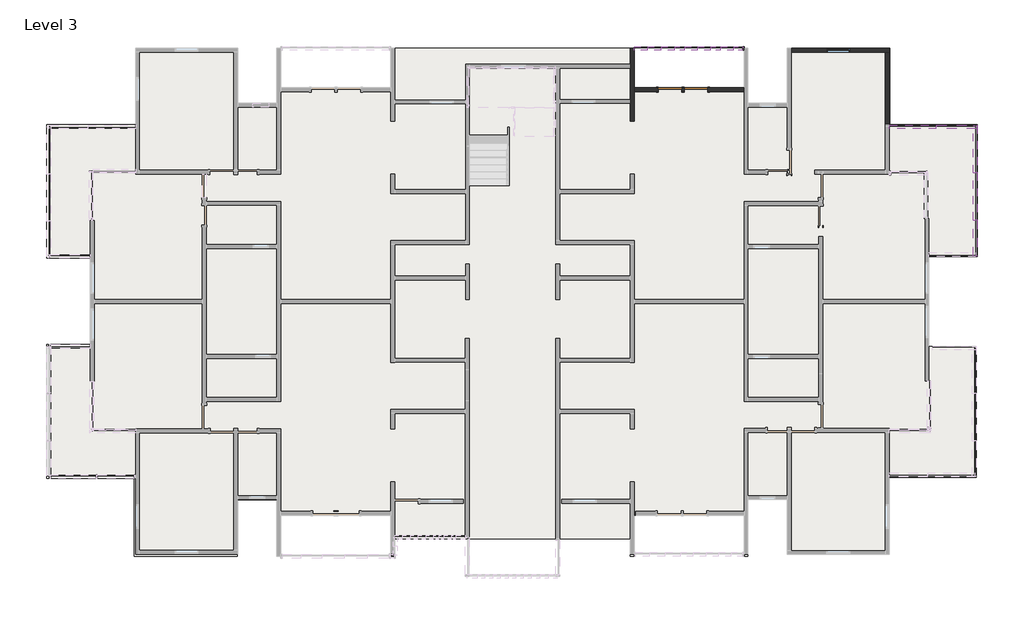
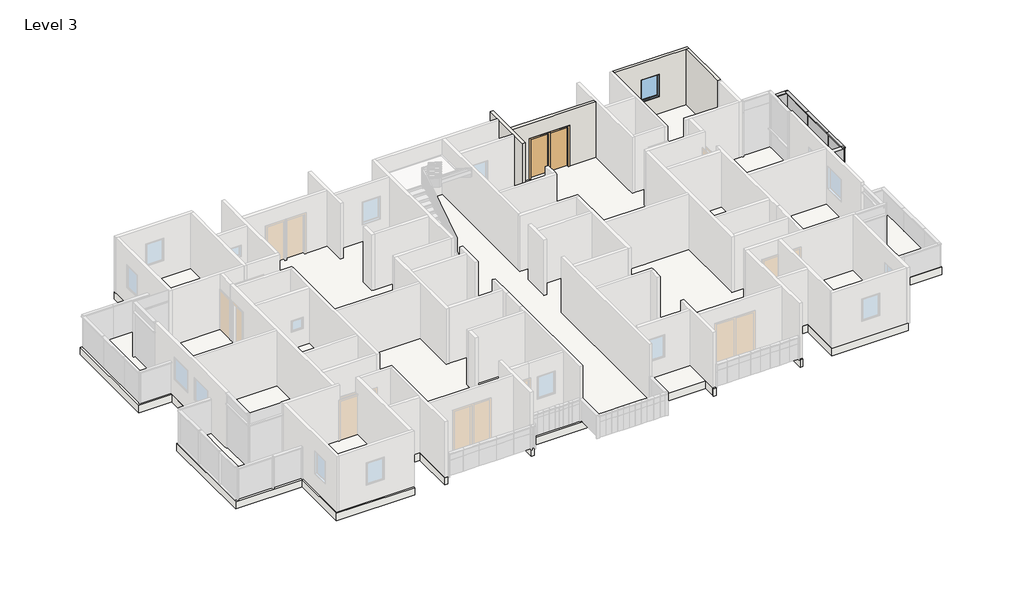
# One storey, part 5 of 7: 15 members, 14 plates, 4 walls, 2 doors, 1 slab, 1 window.
"""IFC4 building model written with IfcOpenShell, lengths in millimetres."""

import ifcopenshell
import ifcopenshell.guid

model = None  # the IFC model being written
_history = None  # IfcOwnerHistory: only IFC2X3 demands one
_inside = {}  # id of a spatial element -> (the spatial element, [elements in it])
_under = {}  # id of a project, library or spatial element -> (it, [spatial elements below it])
_declared = {}  # id of a project -> (the project, [libraries it declares])
_typed = {}  # id of a type object -> (the type object, [elements of that type])
_made_of = {}  # id of a material, layer set ... -> (it, [elements and type objects made of it])


def new_model(schema):
    """Start an empty IFC model of exactly this schema.

    Asked for "IFC4X3", IfcOpenShell would pick the latest addendum, in which some entities
    have other attributes; the version numbers below select the first issue.
    IFC2X3 requires an IfcOwnerHistory on every rooted entity: one is made here for all.
    """
    global model, _history
    if schema == "IFC4X3":
        model = ifcopenshell.file(schema_version=(4, 3, 0, 0))
    else:
        model = ifcopenshell.file(schema=schema)
    _inside.clear()
    _under.clear()
    _declared.clear()
    _typed.clear()
    _made_of.clear()
    _history = None
    if model.schema == "IFC2X3":
        org = make("IfcOrganization", Name="unknown")
        user = make(
            "IfcPersonAndOrganization",
            ThePerson=make("IfcPerson", FamilyName="unknown"),
            TheOrganization=org,
        )
        app = make(
            "IfcApplication",
            ApplicationDeveloper=org,
            Version="unknown",
            ApplicationFullName="unknown",
            ApplicationIdentifier="unknown",
        )
        _history = make(
            "IfcOwnerHistory",
            OwningUser=user,
            OwningApplication=app,
            ChangeAction="ADDED",
            CreationDate=0,
        )
    return model


def make(cls, **values):
    """One entity of the class cls with the attributes given. An attribute that is None is left unset."""
    return model.create_entity(
        cls, **{name: value for name, value in values.items() if value is not None}
    )


def rooted(cls, **values):
    """An entity with a GlobalId (a new one), such as an element, a storey or a relation."""
    return make(cls, GlobalId=ifcopenshell.guid.new(), OwnerHistory=_history, **values)


def si_unit(unit_type, name, prefix=None):
    """IfcSIUnit, for example si_unit("LENGTHUNIT", "METRE", prefix="MILLI")."""
    return make("IfcSIUnit", UnitType=unit_type, Prefix=prefix, Name=name)


def assignment(units):
    """IfcUnitAssignment: the units of a project."""
    return None if units is None else make("IfcUnitAssignment", Units=units)


def point(xyz):
    """IfcCartesianPoint."""
    return None if xyz is None else make("IfcCartesianPoint", Coordinates=xyz)


def direction(xyz):
    """IfcDirection."""
    return None if xyz is None else make("IfcDirection", DirectionRatios=xyz)


def frame(location, z_axis=None, x_axis=None):
    """IfcAxis2Placement3D, a coordinate frame: its origin and axes. An axis left out is left unset."""
    return make(
        "IfcAxis2Placement3D",
        Location=point(location),
        Axis=direction(z_axis),
        RefDirection=direction(x_axis),
    )


def origin():
    """The frame at (0, 0, 0) with its axes left unset."""
    return frame((0.0, 0.0, 0.0))


def origin_with_axes():
    """The frame at (0, 0, 0) with the z axis (0, 0, 1) and the x axis (1, 0, 0) written out."""
    return frame((0.0, 0.0, 0.0), z_axis=(0.0, 0.0, 1.0), x_axis=(1.0, 0.0, 0.0))


def place(relative_to, where):
    """IfcLocalPlacement: puts the frame where relative to a parent placement (None: the world)."""
    return make(
        "IfcLocalPlacement", PlacementRelTo=relative_to, RelativePlacement=where
    )


def context(
    kind, dimensions, precision=None, world=None, true_north=None, identifier=None
):
    """IfcGeometricRepresentationContext, for example the 3D "Model" context."""
    return make(
        "IfcGeometricRepresentationContext",
        ContextIdentifier=identifier,
        ContextType=kind,
        CoordinateSpaceDimension=dimensions,
        Precision=precision,
        WorldCoordinateSystem=world,
        TrueNorth=true_north,
    )


def project(units=None, contexts=None):
    """IfcProject with its units and contexts."""
    return rooted(
        "IfcProject",
        Name="project",
        RepresentationContexts=contexts,
        UnitsInContext=assignment(units),
    )


def spatial(cls, under=None, at=None, **own):
    """A site, building, storey or space (cls), placed at a placement, below another one or the project."""
    s = rooted(cls, ObjectPlacement=at, **own)
    if under is not None:
        _under.setdefault(under.id(), (under, []))[1].append(s)
    return s


def polyline(points):
    """IfcPolyline through the points."""
    return make("IfcPolyline", Points=[point(p) for p in points])


def outline(outer, holes=None, kind="AREA"):
    """IfcArbitraryClosedProfileDef: a profile drawn as a closed curve; with holes, ...WithVoids."""
    if holes is None:
        return make("IfcArbitraryClosedProfileDef", ProfileType=kind, OuterCurve=outer)
    return make(
        "IfcArbitraryProfileDefWithVoids",
        ProfileType=kind,
        OuterCurve=outer,
        InnerCurves=holes,
    )


def extrude(swept, where, along, depth):
    """IfcExtrudedAreaSolid: the profile swept, set in the frame where, extruded along a direction by depth."""
    return make(
        "IfcExtrudedAreaSolid",
        SweptArea=swept,
        Position=where,
        ExtrudedDirection=direction(along),
        Depth=depth,
    )


def faces_of(points, faces, orient=None, outer=None):
    """IfcFace entities. A face is a list of loops; a loop is a list of indices into points, from 0.

    orient and outer hold one flag for each loop. By default every Orientation is true, the
    first loop of a face is its IfcFaceOuterBound and the others are IfcFaceBound.
    """
    made = []
    for i, loops in enumerate(faces):
        bounds = []
        for j, loop in enumerate(loops):
            is_outer = j == 0 if outer is None else outer[i][j]
            bounds.append(
                make(
                    "IfcFaceOuterBound" if is_outer else "IfcFaceBound",
                    Bound=make("IfcPolyLoop", Polygon=[points[k] for k in loop]),
                    Orientation=True if orient is None else orient[i][j],
                )
            )
        made.append(make("IfcFace", Bounds=bounds))
    return made


def faceted_brep(points, faces, orient=None, outer=None, voids=None):
    """IfcFacetedBrep: a solid bounded by flat faces; with voids (closed shells), ...WithVoids."""
    shared = [point(p) for p in points]
    hull = make("IfcClosedShell", CfsFaces=faces_of(shared, faces, orient, outer))
    if voids is None:
        return make("IfcFacetedBrep", Outer=hull)
    return make(
        "IfcFacetedBrepWithVoids",
        Outer=hull,
        Voids=[
            make(cls, CfsFaces=faces_of(shared, fs, o, b)) for cls, fs, o, b in voids
        ],
    )


def shape(context_of_items, identifier, shape_type, items):
    """IfcShapeRepresentation: the items that make up one representation, for example the "Body"."""
    return make(
        "IfcShapeRepresentation",
        ContextOfItems=context_of_items,
        RepresentationIdentifier=identifier,
        RepresentationType=shape_type,
        Items=items,
    )


def source(mapping_origin, context_of_items, identifier, shape_type, items):
    """IfcRepresentationMap: a shape defined once, which mapped items show again and again."""
    return make(
        "IfcRepresentationMap",
        MappingOrigin=mapping_origin,
        MappedRepresentation=shape(context_of_items, identifier, shape_type, items),
    )


def transform(
    local_origin,
    x_axis=None,
    y_axis=None,
    z_axis=None,
    scale=None,
    scale2=None,
    scale3=None,
    uniform=True,
):
    """IfcCartesianTransformationOperator3D, or its non-uniform kind. x_axis, y_axis, z_axis: its Axis1, 2, 3."""
    if uniform:
        return make(
            "IfcCartesianTransformationOperator3D",
            Axis1=direction(x_axis),
            Axis2=direction(y_axis),
            LocalOrigin=point(local_origin),
            Scale=scale,
            Axis3=direction(z_axis),
        )
    return make(
        "IfcCartesianTransformationOperator3DnonUniform",
        Axis1=direction(x_axis),
        Axis2=direction(y_axis),
        LocalOrigin=point(local_origin),
        Scale=scale,
        Axis3=direction(z_axis),
        Scale2=scale2,
        Scale3=scale3,
    )


def mapped(mapping_source, mapping_target):
    """IfcMappedItem: shows the shape of a source again, moved by a transform."""
    return make(
        "IfcMappedItem", MappingSource=mapping_source, MappingTarget=mapping_target
    )


def made_of(thing, what):
    """Note that an element or type object is made of a material, layer set ...; save() writes the relation."""
    if what is not None:
        _made_of.setdefault(what.id(), (what, []))[1].append(thing)
    return thing


def element(
    cls,
    number,
    at=None,
    inside=None,
    cuts=None,
    type_object=None,
    material=None,
    context=None,
    identifier="Body",
    shape_type=None,
    held_by="IfcProductDefinitionShape",
    body=None,
    shapes=None,
    **own,
):
    """One element of the class cls, such as IfcWall. Its Tag is "e" and its number.

    at: its placement. inside: the storey or other place that contains it. cuts: it is an
    opening in that element (IfcRelVoidsElement). A single representation is given by context,
    identifier, shape_type and body (its items); several are given by shapes. held_by: the class
    of the entity that holds the representations. save() writes the other relations.
    """
    e = rooted(cls, Tag="e%d" % number, ObjectPlacement=at, **own)
    if body is not None:
        shapes = [shape(context, identifier, shape_type, body)]
    if shapes is not None:
        e.Representation = make(held_by, Representations=shapes)
    if inside is not None:
        _inside.setdefault(inside.id(), (inside, []))[1].append(e)
    if cuts is not None:
        rooted(
            "IfcRelVoidsElement", RelatingBuildingElement=cuts, RelatedOpeningElement=e
        )
    if type_object is not None:
        _typed.setdefault(type_object.id(), (type_object, []))[1].append(e)
    return made_of(e, material)


def aggregate(whole, parts):
    """IfcRelAggregates: a whole, such as a stair, and the parts it consists of."""
    return rooted("IfcRelAggregates", RelatingObject=whole, RelatedObjects=parts)


def save(model, path):
    """Write the relations noted so far, then the file.

    IfcRelAggregates (storeys below a building ...), IfcRelContainedInSpatialStructure (elements
    in a storey), IfcRelDefinesByType, IfcRelAssociatesMaterial and IfcRelDeclares: one each for
    every whole, place, type object, material and project.
    """
    for whole, parts in _under.values():
        aggregate(whole, parts)
    for where, things in _inside.values():
        rooted(
            "IfcRelContainedInSpatialStructure",
            RelatedElements=things,
            RelatingStructure=where,
        )
    for kind, things in _typed.values():
        rooted("IfcRelDefinesByType", RelatedObjects=things, RelatingType=kind)
    for what, things in _made_of.values():
        rooted("IfcRelAssociatesMaterial", RelatedObjects=things, RelatingMaterial=what)
    for by, libraries in _declared.values():
        rooted("IfcRelDeclares", RelatingContext=by, RelatedDefinitions=libraries)
    model.write(path)


def m_single_flush_0915_x_2134mm_138fd904(model_context):
    return source(origin(), model_context, "Body", "SweptSolid", [
        extrude(outline(polyline([(2210.0, -533.5), (0.0, -533.5), (0.0, -457.5), (2134.0, -457.5), (2134.0, 457.5), (0.0, 457.5), (0.0, 533.5), (2210.0, 533.5), (2210.0, -533.5)])), frame((0.0, 75.0, 0.0), z_axis=(0.0, 1.0, 0.0), x_axis=(0.0, 0.0, 1.0)), (0.0, 0.0, 1.0), 25.0),
        extrude(outline(polyline([(2210.0, 533.5), (2210.0, -533.5), (0.0, -533.5), (0.0, -457.5), (2134.0, -457.5), (2134.0, 457.5), (0.0, 457.5), (0.0, 533.5), (2210.0, 533.5)])), frame((0.0, -100.0, 0.0), z_axis=(0.0, 1.0, 0.0), x_axis=(0.0, 0.0, 1.0)), (0.0, 0.0, 1.0), 25.0),
        extrude(outline(polyline([(457.5, 24.0), (-457.5, 24.0), (-457.5, 75.0), (457.5, 75.0), (457.5, 24.0)])), origin_with_axes(), (0.0, 0.0, 1.0), 2134.0),
    ])


def rectangular_mullion_50mm_x_150mm_42770ee2(model_context):
    return source(origin(), model_context, "Body", "SweptSolid", [
        extrude(outline(polyline([(0.0, 75.0), (0.0, -75.0), (-50.0, -75.0), (-50.0, 75.0), (0.0, 75.0)])), frame((0.0, 0.0, -1830.0000003), z_axis=(0.0, 0.0, 1.0), x_axis=(1.0, 0.0, 0.0)), (0.0, 0.0, 1.0), 1830.0000003),
    ])


def rectangular_mullion_50mm_x_150mm_aaee7d48(model_context):
    return source(origin(), model_context, "Body", "SweptSolid", [
        extrude(outline(polyline([(0.0, 75.0), (0.0, -75.0), (-50.0, -75.0), (-50.0, 75.0), (0.0, 75.0)])), frame((0.0, 0.0, -1830.0), z_axis=(0.0, 0.0, 1.0), x_axis=(1.0, 0.0, 0.0)), (0.0, 0.0, 1.0), 1830.0),
    ])


def rectangular_mullion_50mm_x_150mm_efa02866(model_context):
    return source(origin(), model_context, "Body", "SweptSolid", [
        extrude(outline(polyline([(0.0, 75.0), (0.0, -75.0), (-50.0, -75.0), (-50.0, 75.0), (0.0, 75.0)])), frame((0.0, 0.0, -1399.9999997), z_axis=(0.0, 0.0, 1.0), x_axis=(1.0, 0.0, 0.0)), (0.0, 0.0, 1.0), 1399.9999997),
    ])


def rectangular_mullion_50mm_x_150mm_d9f1e9e9(model_context):
    return source(origin(), model_context, "Body", "SweptSolid", [
        extrude(outline(polyline([(0.0, 75.0), (0.0, -75.0), (-50.0, -75.0), (-50.0, 75.0), (0.0, 75.0)])), frame((0.0, 0.0, -1565.8160321), z_axis=(0.0, 0.0, 1.0), x_axis=(1.0, 0.0, 0.0)), (0.0, 0.0, 1.0), 1565.8160321),
    ])


def rectangular_mullion_50mm_x_150mm_729c0cfc(model_context):
    return source(origin(), model_context, "Body", "SweptSolid", [
        extrude(outline(polyline([(0.0, 75.0), (0.0, -75.0), (-50.0, -75.0), (-50.0, 75.0), (0.0, 75.0)])), frame((0.0, 0.0, -1250.0), z_axis=(0.0, 0.0, 1.0), x_axis=(1.0, 0.0, 0.0)), (0.0, 0.0, 1.0), 1250.0),
    ])


def rectangular_mullion_50mm_x_150mm_b3666dbd(model_context):
    return source(origin(), model_context, "Body", "SweptSolid", [
        extrude(outline(polyline([(0.0, 75.0), (0.0, -75.0), (-50.0, -75.0), (-50.0, 75.0), (0.0, 75.0)])), frame((0.0, 0.0, -500.0), z_axis=(0.0, 0.0, 1.0), x_axis=(1.0, 0.0, 0.0)), (0.0, 0.0, 1.0), 500.0),
    ])


def rectangular_mullion_50mm_x_150mm_e851a0b8(model_context):
    return source(origin(), model_context, "Body", "SweptSolid", [
        extrude(outline(polyline([(0.0, 75.0), (0.0, -75.0), (-50.0, -75.0), (-50.0, 75.0), (0.0, 75.0)])), frame((0.0, 0.0, -522.7272727), z_axis=(0.0, 0.0, 1.0), x_axis=(1.0, 0.0, 0.0)), (0.0, 0.0, 1.0), 522.7272727),
    ])


def rectangular_mullion_50mm_x_150mm_e11a3e7b(model_context):
    return source(origin(), model_context, "Body", "SweptSolid", [
        extrude(outline(polyline([(0.0, 75.0), (0.0, -75.0), (-50.0, -75.0), (-50.0, 75.0), (0.0, 75.0)])), frame((0.0, 0.0, -400.0), z_axis=(0.0, 0.0, 1.0), x_axis=(1.0, 0.0, 0.0)), (0.0, 0.0, 1.0), 400.0),
    ])


def rectangular_mullion_50mm_x_150mm_23485ade(model_context):
    return source(origin(), model_context, "Body", "SweptSolid", [
        extrude(outline(polyline([(0.0, 75.0), (0.0, -75.0), (-50.0, -75.0), (-50.0, 75.0), (0.0, 75.0)])), frame((0.0, 0.0, -350.0), z_axis=(0.0, 0.0, 1.0), x_axis=(1.0, 0.0, 0.0)), (0.0, 0.0, 1.0), 350.0),
    ])


def system_panel_glazed_09fbcc53(model_context):
    return source(origin(), model_context, "Body", "SweptSolid", [
        extrude(outline(polyline([(915.0000002, 24.5), (-915.0000002, 24.5), (-915.0000002, 49.5), (915.0000002, 49.5), (915.0000002, 24.5)])), origin_with_axes(), (0.0, 0.0, 1.0), 1200.0),
    ])


def system_panel_glazed_f4bbd109(model_context):
    return source(origin(), model_context, "Body", "SweptSolid", [
        extrude(outline(polyline([(910.8343113, 24.5), (-910.8343113, 24.5), (-910.8343113, 49.5), (910.8343113, 49.5), (910.8343113, 24.5)])), origin_with_axes(), (0.0, 0.0, 1.0), 1200.0),
    ])


def system_panel_glazed_42eec186(model_context):
    return source(origin(), model_context, "Body", "SweptSolid", [
        extrude(outline(polyline([(699.9999998, 24.5), (-699.9999998, 24.5), (-699.9999998, 49.5), (699.9999998, 49.5), (699.9999998, 24.5)])), origin_with_axes(), (0.0, 0.0, 1.0), 1200.0),
    ])


def system_panel_glazed_f2fc581d(model_context):
    return source(origin(), model_context, "Body", "SweptSolid", [
        extrude(outline(polyline([(782.9080161, 24.5), (-782.9080161, 24.5), (-782.9080161, 49.5), (782.9080161, 49.5), (782.9080161, 24.5)])), origin_with_axes(), (0.0, 0.0, 1.0), 1200.0),
    ])


def system_panel_glazed_346501af(model_context):
    return source(origin(), model_context, "Body", "SweptSolid", [
        extrude(outline(polyline([(250.0, 24.5), (-250.0, 24.5), (-250.0, 49.5), (250.0, 49.5), (250.0, 24.5)])), origin_with_axes(), (0.0, 0.0, 1.0), 1200.0),
    ])


def system_panel_glazed_5241e6d5(model_context):
    return source(origin(), model_context, "Body", "SweptSolid", [
        extrude(outline(polyline([(261.3636364, 24.5), (-261.3636364, 24.5), (-261.3636364, 49.5), (261.3636364, 49.5), (261.3636364, 24.5)])), origin_with_axes(), (0.0, 0.0, 1.0), 1200.0),
    ])


def system_panel_glazed_3e660766(model_context):
    return source(origin(), model_context, "Body", "SweptSolid", [
        extrude(outline(polyline([(200.0, 24.5), (-200.0, 24.5), (-200.0, 49.5), (200.0, 49.5), (200.0, 24.5)])), origin_with_axes(), (0.0, 0.0, 1.0), 1200.0),
    ])


def system_panel_glazed_b0a6d7cd(model_context):
    return source(origin(), model_context, "Body", "SweptSolid", [
        extrude(outline(polyline([(175.0, 24.5), (-175.0, 24.5), (-175.0, 49.5), (175.0, 49.5), (175.0, 24.5)])), origin_with_axes(), (0.0, 0.0, 1.0), 1200.0),
    ])


def m_fixed_0915_x_1220mm_873aa0e2(model_context):
    return source(origin(), model_context, "Body", "SweptSolid", [
        extrude(outline(polyline([(-394.5, 53.0), (394.5, 53.0), (394.5, 41.0), (-394.5, 41.0), (-394.5, 53.0)])), frame((0.0, 0.0, 978.0), z_axis=(0.0, 0.0, 1.0), x_axis=(1.0, 0.0, 0.0)), (0.0, 0.0, 1.0), 1094.0),
        extrude(outline(polyline([(2116.0, -438.5), (934.0, -438.5), (934.0, 438.5), (2116.0, 438.5), (2116.0, -438.5)]), holes=[polyline([(2072.0, -394.5), (2072.0, 394.5), (978.0, 394.5), (978.0, -394.5), (2072.0, -394.5)])]), frame((0.0, 25.0, 0.0), z_axis=(0.0, 1.0, 0.0), x_axis=(0.0, 0.0, 1.0)), (0.0, 0.0, 1.0), 44.0),
        extrude(outline(polyline([(2135.0, -457.5), (915.0, -457.5), (915.0, 457.5), (2135.0, 457.5), (2135.0, -457.5)]), holes=[polyline([(2116.0, -438.5), (2116.0, 438.5), (934.0, 438.5), (934.0, -438.5), (2116.0, -438.5)])]), frame((0.0, 25.0, 0.0), z_axis=(0.0, 1.0, 0.0), x_axis=(0.0, 0.0, 1.0)), (0.0, 0.0, 1.0), 63.0),
        extrude(outline(polyline([(2135.0, -457.5), (915.0, -457.5), (915.0, 457.5), (2135.0, 457.5), (2135.0, -457.5)]), holes=[polyline([(2103.0, -425.5), (2103.0, 425.5), (947.0, 425.5), (947.0, -425.5), (2103.0, -425.5)])]), frame((0.0, -62.0, 0.0), z_axis=(0.0, 1.0, 0.0), x_axis=(0.0, 0.0, 1.0)), (0.0, 0.0, 1.0), 87.0),
    ])


model = new_model("IFC4")

# Units and contexts
model_context = context("Model", 3, world=origin())
ifc_project = project(units=[si_unit("LENGTHUNIT", "METRE", prefix="MILLI")], contexts=[model_context])

# Site, building, storey
site = spatial("IfcSite", under=ifc_project)
building = spatial("IfcBuilding", under=site)
storey = spatial("IfcBuildingStorey", under=building, Name="Level 3", Elevation=6500.0)

# Doors
placement = place(None, origin())
m_single_flush_0915_x_2134mm_shape = m_single_flush_0915_x_2134mm_138fd904(model_context)
element("IfcDoor", 1, ObjectType="M_Single-Flush : 0915 x 2134mm", at=placement, inside=storey, context=model_context, shape_type="MappedRepresentation", body=[
    mapped(m_single_flush_0915_x_2134mm_shape, transform((6794.6515415, 8016.5690894, 6500.0), x_axis=(1.0, 0.0, 0.0), y_axis=(0.0, 1.0, 0.0), z_axis=(0.0, 0.0, 1.0))),
])
element("IfcDoor", 2, ObjectType="M_Single-Flush : 0915 x 2134mm", at=placement, inside=storey, context=model_context, shape_type="MappedRepresentation", body=[
    mapped(m_single_flush_0915_x_2134mm_shape, transform((5794.6515415, 8016.5690894, 6500.0), x_axis=(1.0, 0.0, 0.0), y_axis=(0.0, 1.0, 0.0), z_axis=(0.0, 0.0, 1.0))),
])

# Members
rectangular_mullion_50mm_x_150mm_shape = rectangular_mullion_50mm_x_150mm_42770ee2(model_context)
element("IfcMember", 3, ObjectType="Rectangular Mullion : 50mm x 150mm", at=placement, inside=storey, context=model_context, shape_type="MappedRepresentation", body=[
    mapped(rectangular_mullion_50mm_x_150mm_shape, transform((17635.0130284, 4788.3418163, 7750.0), x_axis=(0.0, 0.0, 1.0), y_axis=(-1.0, 0.0, 0.0), z_axis=(0.0, -1.0, 0.0))),
])
element("IfcMember", 4, ObjectType="Rectangular Mullion : 50mm x 150mm", at=placement, inside=storey, context=model_context, shape_type="MappedRepresentation", body=[
    mapped(rectangular_mullion_50mm_x_150mm_shape, transform((16129.1969963, 6568.8418166, 7750.0), x_axis=(0.0, 0.0, 1.0), y_axis=(0.0, -1.0, 0.0), z_axis=(1.0, 0.0, 0.0))),
])
rectangular_mullion_50mm_x_150mm_2_shape = rectangular_mullion_50mm_x_150mm_aaee7d48(model_context)
element("IfcMember", 5, ObjectType="Rectangular Mullion : 50mm x 150mm", at=placement, inside=storey, context=model_context, shape_type="MappedRepresentation", body=[
    mapped(rectangular_mullion_50mm_x_150mm_2_shape, transform((17635.0130284, 2958.3418163, 7750.0), x_axis=(0.0, 0.0, 1.0), y_axis=(-1.0, 0.0, 0.0), z_axis=(0.0, -1.0, 0.0))),
])
rectangular_mullion_50mm_x_150mm_3_shape = rectangular_mullion_50mm_x_150mm_efa02866(model_context)
element("IfcMember", 6, ObjectType="Rectangular Mullion : 50mm x 150mm", at=placement, inside=storey, context=model_context, shape_type="MappedRepresentation", body=[
    mapped(rectangular_mullion_50mm_x_150mm_3_shape, transform((17635.0130284, 1558.3418166, 7750.0), x_axis=(0.0, 0.0, 1.0), y_axis=(-1.0, 0.0, 0.0), z_axis=(0.0, -1.0, 0.0))),
])
rectangular_mullion_50mm_x_150mm_4_shape = rectangular_mullion_50mm_x_150mm_d9f1e9e9(model_context)
element("IfcMember", 7, ObjectType="Rectangular Mullion : 50mm x 150mm", at=placement, inside=storey, context=model_context, shape_type="MappedRepresentation", body=[
    mapped(rectangular_mullion_50mm_x_150mm_4_shape, transform((17695.0130284, 6568.8418166, 7750.0), x_axis=(0.0, 0.0, 1.0), y_axis=(0.0, -1.0, 0.0), z_axis=(1.0, 0.0, 0.0))),
])
rectangular_mullion_50mm_x_150mm_5_shape = rectangular_mullion_50mm_x_150mm_729c0cfc(model_context)
element("IfcMember", 8, ObjectType="Rectangular Mullion : 50mm x 150mm", at=placement, inside=storey, context=model_context, shape_type="MappedRepresentation", body=[
    mapped(rectangular_mullion_50mm_x_150mm_5_shape, transform((8667.3788142, 9614.2963621, 6500.0), x_axis=(1.0, 0.0, 0.0), y_axis=(0.0, -1.0, 0.0), z_axis=(0.0, 0.0, -1.0))),
])
rectangular_mullion_50mm_x_150mm_6_shape = rectangular_mullion_50mm_x_150mm_b3666dbd(model_context)
element("IfcMember", 9, ObjectType="Rectangular Mullion : 50mm x 150mm", at=placement, inside=storey, context=model_context, shape_type="MappedRepresentation", body=[
    mapped(rectangular_mullion_50mm_x_150mm_6_shape, transform((6867.3788142, 9614.2963621, 7750.0), x_axis=(0.0, 0.0, 1.0), y_axis=(0.0, -1.0, 0.0), z_axis=(1.0, 0.0, 0.0))),
])
element("IfcMember", 10, ObjectType="Rectangular Mullion : 50mm x 150mm", at=placement, inside=storey, context=model_context, shape_type="MappedRepresentation", body=[
    mapped(rectangular_mullion_50mm_x_150mm_6_shape, transform((7367.3788142, 9614.2963621, 7750.0), x_axis=(0.0, 0.0, 1.0), y_axis=(0.0, -1.0, 0.0), z_axis=(1.0, 0.0, 0.0))),
])
element("IfcMember", 11, ObjectType="Rectangular Mullion : 50mm x 150mm", at=placement, inside=storey, context=model_context, shape_type="MappedRepresentation", body=[
    mapped(rectangular_mullion_50mm_x_150mm_6_shape, transform((8267.3788142, 9614.2963621, 7750.0), x_axis=(0.0, 0.0, 1.0), y_axis=(0.0, -1.0, 0.0), z_axis=(1.0, 0.0, 0.0))),
])
rectangular_mullion_50mm_x_150mm_7_shape = rectangular_mullion_50mm_x_150mm_e851a0b8(model_context)
element("IfcMember", 12, ObjectType="Rectangular Mullion : 50mm x 150mm", at=placement, inside=storey, context=model_context, shape_type="MappedRepresentation", body=[
    mapped(rectangular_mullion_50mm_x_150mm_7_shape, transform((4921.9242687, 9614.2963621, 7750.0), x_axis=(0.0, 0.0, 1.0), y_axis=(0.0, -1.0, 0.0), z_axis=(1.0, 0.0, 0.0))),
])
element("IfcMember", 13, ObjectType="Rectangular Mullion : 50mm x 150mm", at=placement, inside=storey, context=model_context, shape_type="MappedRepresentation", body=[
    mapped(rectangular_mullion_50mm_x_150mm_7_shape, transform((5444.6515415, 9614.2963621, 7750.0), x_axis=(0.0, 0.0, 1.0), y_axis=(0.0, -1.0, 0.0), z_axis=(1.0, 0.0, 0.0))),
])
element("IfcMember", 14, ObjectType="Rectangular Mullion : 50mm x 150mm", at=placement, inside=storey, context=model_context, shape_type="MappedRepresentation", body=[
    mapped(rectangular_mullion_50mm_x_150mm_7_shape, transform((5967.3788142, 9614.2963621, 7750.0), x_axis=(0.0, 0.0, 1.0), y_axis=(0.0, -1.0, 0.0), z_axis=(1.0, 0.0, 0.0))),
])
rectangular_mullion_50mm_x_150mm_8_shape = rectangular_mullion_50mm_x_150mm_e11a3e7b(model_context)
element("IfcMember", 15, ObjectType="Rectangular Mullion : 50mm x 150mm", at=placement, inside=storey, context=model_context, shape_type="MappedRepresentation", body=[
    mapped(rectangular_mullion_50mm_x_150mm_8_shape, transform((6367.3788142, 9614.2963621, 7750.0), x_axis=(0.0, 0.0, 1.0), y_axis=(0.0, -1.0, 0.0), z_axis=(1.0, 0.0, 0.0))),
])
element("IfcMember", 16, ObjectType="Rectangular Mullion : 50mm x 150mm", at=placement, inside=storey, context=model_context, shape_type="MappedRepresentation", body=[
    mapped(rectangular_mullion_50mm_x_150mm_8_shape, transform((7767.3788142, 9614.2963621, 7750.0), x_axis=(0.0, 0.0, 1.0), y_axis=(0.0, -1.0, 0.0), z_axis=(1.0, 0.0, 0.0))),
])
rectangular_mullion_50mm_x_150mm_9_shape = rectangular_mullion_50mm_x_150mm_23485ade(model_context)
element("IfcMember", 17, ObjectType="Rectangular Mullion : 50mm x 150mm", at=placement, inside=storey, context=model_context, shape_type="MappedRepresentation", body=[
    mapped(rectangular_mullion_50mm_x_150mm_9_shape, transform((8617.3788142, 9614.2963621, 7750.0), x_axis=(0.0, 0.0, 1.0), y_axis=(0.0, -1.0, 0.0), z_axis=(1.0, 0.0, 0.0))),
])

# Plates
system_panel_glazed_shape = system_panel_glazed_09fbcc53(model_context)
element("IfcPlate", 18, ObjectType="System Panel : Glazed", at=placement, inside=storey, context=model_context, shape_type="MappedRepresentation", body=[
    mapped(system_panel_glazed_shape, transform((17635.0130284, 5703.3418165, 6500.0), x_axis=(0.0, -1.0, 0.0), y_axis=(1.0, 0.0, 0.0), z_axis=(0.0, 0.0, 1.0))),
])
element("IfcPlate", 19, ObjectType="System Panel : Glazed", at=placement, inside=storey, context=model_context, shape_type="MappedRepresentation", body=[
    mapped(system_panel_glazed_shape, transform((17635.0130284, 3873.3418163, 6500.0), x_axis=(0.0, -1.0, 0.0), y_axis=(1.0, 0.0, 0.0), z_axis=(0.0, 0.0, 1.0))),
])
system_panel_glazed_2_shape = system_panel_glazed_f4bbd109(model_context)
element("IfcPlate", 20, ObjectType="System Panel : Glazed", at=placement, inside=storey, context=model_context, shape_type="MappedRepresentation", body=[
    mapped(system_panel_glazed_2_shape, transform((16748.6787171, 1608.3418166, 6500.0), x_axis=(-1.0, 0.0, 0.0), y_axis=(0.0, -1.0, 0.0), z_axis=(0.0, 0.0, 1.0))),
])
system_panel_glazed_3_shape = system_panel_glazed_42eec186(model_context)
element("IfcPlate", 21, ObjectType="System Panel : Glazed", at=placement, inside=storey, context=model_context, shape_type="MappedRepresentation", body=[
    mapped(system_panel_glazed_3_shape, transform((17635.0130284, 2258.3418165, 6500.0), x_axis=(0.0, -1.0, 0.0), y_axis=(1.0, 0.0, 0.0), z_axis=(0.0, 0.0, 1.0))),
])
system_panel_glazed_4_shape = system_panel_glazed_f2fc581d(model_context)
element("IfcPlate", 22, ObjectType="System Panel : Glazed", at=placement, inside=storey, context=model_context, shape_type="MappedRepresentation", body=[
    mapped(system_panel_glazed_4_shape, transform((16912.1050124, 6568.8418166, 6500.0), x_axis=(1.0, 0.0, 0.0), y_axis=(0.0, 1.0, 0.0), z_axis=(0.0, 0.0, 1.0))),
])
system_panel_glazed_5_shape = system_panel_glazed_346501af(model_context)
element("IfcPlate", 23, ObjectType="System Panel : Glazed", at=placement, inside=storey, context=model_context, shape_type="MappedRepresentation", body=[
    mapped(system_panel_glazed_5_shape, transform((8017.3788142, 9614.2963621, 6500.0), x_axis=(1.0, 0.0, 0.0), y_axis=(0.0, 1.0, 0.0), z_axis=(0.0, 0.0, 1.0))),
])
element("IfcPlate", 24, ObjectType="System Panel : Glazed", at=placement, inside=storey, context=model_context, shape_type="MappedRepresentation", body=[
    mapped(system_panel_glazed_5_shape, transform((7117.3788142, 9614.2963621, 6500.0), x_axis=(1.0, 0.0, 0.0), y_axis=(0.0, 1.0, 0.0), z_axis=(0.0, 0.0, 1.0))),
])
element("IfcPlate", 25, ObjectType="System Panel : Glazed", at=placement, inside=storey, context=model_context, shape_type="MappedRepresentation", body=[
    mapped(system_panel_glazed_5_shape, transform((6617.3788142, 9614.2963621, 6500.0), x_axis=(1.0, 0.0, 0.0), y_axis=(0.0, 1.0, 0.0), z_axis=(0.0, 0.0, 1.0))),
])
system_panel_glazed_6_shape = system_panel_glazed_5241e6d5(model_context)
element("IfcPlate", 26, ObjectType="System Panel : Glazed", at=placement, inside=storey, context=model_context, shape_type="MappedRepresentation", body=[
    mapped(system_panel_glazed_6_shape, transform((4660.5606324, 9614.2963621, 6500.0), x_axis=(1.0, 0.0, 0.0), y_axis=(0.0, 1.0, 0.0), z_axis=(0.0, 0.0, 1.0))),
])
element("IfcPlate", 27, ObjectType="System Panel : Glazed", at=placement, inside=storey, context=model_context, shape_type="MappedRepresentation", body=[
    mapped(system_panel_glazed_6_shape, transform((5706.0151778, 9614.2963621, 6500.0), x_axis=(1.0, 0.0, 0.0), y_axis=(0.0, 1.0, 0.0), z_axis=(0.0, 0.0, 1.0))),
])
element("IfcPlate", 28, ObjectType="System Panel : Glazed", at=placement, inside=storey, context=model_context, shape_type="MappedRepresentation", body=[
    mapped(system_panel_glazed_6_shape, transform((5183.2879051, 9614.2963621, 6500.0), x_axis=(1.0, 0.0, 0.0), y_axis=(0.0, 1.0, 0.0), z_axis=(0.0, 0.0, 1.0))),
])
system_panel_glazed_7_shape = system_panel_glazed_3e660766(model_context)
element("IfcPlate", 29, ObjectType="System Panel : Glazed", at=placement, inside=storey, context=model_context, shape_type="MappedRepresentation", body=[
    mapped(system_panel_glazed_7_shape, transform((7567.3788142, 9614.2963621, 6500.0), x_axis=(1.0, 0.0, 0.0), y_axis=(0.0, 1.0, 0.0), z_axis=(0.0, 0.0, 1.0))),
])
element("IfcPlate", 30, ObjectType="System Panel : Glazed", at=placement, inside=storey, context=model_context, shape_type="MappedRepresentation", body=[
    mapped(system_panel_glazed_7_shape, transform((6167.3788142, 9614.2963621, 6500.0), x_axis=(1.0, 0.0, 0.0), y_axis=(0.0, 1.0, 0.0), z_axis=(0.0, 0.0, 1.0))),
])
system_panel_glazed_8_shape = system_panel_glazed_b0a6d7cd(model_context)
element("IfcPlate", 31, ObjectType="System Panel : Glazed", at=placement, inside=storey, context=model_context, shape_type="MappedRepresentation", body=[
    mapped(system_panel_glazed_8_shape, transform((8442.3788142, 9614.2963621, 6500.0), x_axis=(1.0, 0.0, 0.0), y_axis=(0.0, 1.0, 0.0), z_axis=(0.0, 0.0, 1.0))),
])

# Slab
element("IfcSlab", 32, ObjectType="Generic Floor - 400mm", at=placement, inside=storey, context=model_context, shape_type="SweptSolid", body=[
    extrude(outline(polyline([(-10978.0757313, 7482.4781803), (-9455.3484585, 7482.4781803), (-9455.3484585, 9614.2963621), (-9305.3484585, 9614.2963621), (-9305.3484585, 8091.5690894), (-5039.4393676, 8091.5690894), (-5039.4393676, 9614.2963621), (4399.196996, 9614.2963621), (4399.196996, 8091.5690894), (8665.1060869, 8091.5690894), (8665.1060869, 9614.2963621), (8817.3788142, 9614.2963621), (8817.3788142, 7482.4781803), (10342.3783683, 7482.4781803), (10342.3783683, 9614.2963621), (14312.8444058, 9614.2963621), (14312.8444058, 6653.3418166), (17717.8444058, 6653.3418166), (17717.8444058, 1533.3418166), (15837.8444058, 1533.3418166), (15837.8444058, -1946.1581834), (17677.8444058, -1946.1581834), (17677.8444058, -7028.8854561), (14240.1060869, -7028.8854561), (14240.1060869, -10028.8854561), (10340.1060869, -10028.8854561), (10340.1060869, -7894.794547), (8815.1060869, -7894.794547), (8815.1060869, -10106.1581834), (8665.1060869, -10106.1581834), (8665.1060869, -8506.1581834), (4401.4697233, -8506.1581834), (4401.4697233, -10106.1581834), (4251.4697233, -10106.1581834), (4251.4697233, -10028.8854561), (4251.4697233, -9417.5218198), (-4887.1666404, -9417.5218198), (-4887.1666404, -10006.7413208), (-4887.1666404, -10106.1581834), (-5039.4393676, -10106.1581834), (-5039.4393676, -8503.8854561), (-9303.0757313, -8503.8854561), (-9303.0757313, -10106.1581834), (-9453.0757313, -10106.1581834), (-9453.0757313, -7906.1581834), (-10989.3512663, -7906.1581834), (-10989.3512663, -10106.1581834), (-14989.3512663, -10106.1581834), (-14989.3512663, -7083.4309107), (-18389.3512663, -7083.4309107), (-18389.3512663, -1883.4309107), (-16697.1666404, -1883.4309107), (-16697.1666404, 1474.2963621), (-18377.1666404, 1474.2963621), (-18377.1666404, 6654.2963621), (-14937.1666404, 6654.2963621), (-14937.1666404, 9614.2963621), (-10978.0757313, 9614.2963621), (-10978.0757313, 7482.4781803)])), frame((0.0, 0.0, 6100.0), z_axis=(0.0, 0.0, 1.0), x_axis=(1.0, 0.0, 0.0)), (0.0, 0.0, 1.0), 400.0),
])

# Walls
element("IfcWall", 33, ObjectType="wal 150", at=placement, inside=storey, context=model_context, shape_type="Brep", body=[
    faceted_brep([(4399.196996, 6792.1522268, 6500.0), (4399.196996, 7941.5690894, 6500.0), (4399.196996, 8091.5690894, 6500.0), (4399.196996, 9614.2963621, 6500.0), (4399.196996, 9614.2963621, 9500.0), (4399.196996, 8091.5690894, 9500.0), (4399.196996, 7941.5690894, 9500.0), (4399.196996, 6792.1522268, 9500.0), (4249.196996, 6792.1522268, 6500.0), (4249.196996, 6792.1522268, 9500.0), (4249.196996, 7484.7509075, 9500.0), (4249.196996, 7634.7509075, 9500.0), (4249.196996, 8855.205453, 9500.0), (4249.196996, 9005.205453, 9500.0), (4249.196996, 9614.2963621, 9500.0), (4249.196996, 9614.2963621, 6500.0), (4249.196996, 9005.205453, 6500.0), (4249.196996, 8855.205453, 6500.0), (4249.196996, 7634.7509075, 6500.0), (4249.196996, 7484.7509075, 6500.0)], [[[0, 1, 2, 3, 4, 5, 6, 7]], [[8, 9, 10, 11, 12, 13, 14, 15, 16, 17, 18, 19]], [[3, 2, 1, 0, 8, 19, 18, 17, 16, 15]], [[4, 3, 15, 14]], [[7, 6, 5, 4, 14, 13, 12, 11, 10, 9]], [[0, 7, 9, 8]]]),
])
element("IfcWall", 34, ObjectType="wal 150", at=placement, inside=storey, context=model_context, shape_type="SweptSolid", body=[
    extrude(outline(polyline([(6500.0, 8665.1060869), (9500.0, 8665.1060869), (9500.0, 4399.196996), (6500.0, 4399.196996), (6500.0, 5337.1515415), (8634.0, 5337.1515415), (8634.0, 6252.1515415), (6500.0, 6252.1515415), (6500.0, 6337.1515415), (8634.0, 6337.1515415), (8634.0, 7252.1515415), (6500.0, 7252.1515415), (6500.0, 8665.1060869)])), frame((0.0, 7941.5690894, 0.0), z_axis=(0.0, 1.0, 0.0), x_axis=(0.0, 0.0, 1.0)), (0.0, 0.0, 1.0), 150.0),
])
element("IfcWall", 35, ObjectType="wal 150", at=placement, inside=storey, context=model_context, shape_type="Brep", body=[
    faceted_brep([(10492.3783683, 9464.2963621, 6500.0), (14149.196996, 9464.2963621, 6500.0), (14299.196996, 9464.2963621, 6500.0), (14299.196996, 9464.2963621, 9500.0), (14149.196996, 9464.2963621, 9500.0), (10492.3783683, 9464.2963621, 9500.0), (11863.2876822, 9464.2963621, 7415.0), (11863.2876822, 9464.2963621, 8635.0), (12778.2876822, 9464.2963621, 8635.0), (12778.2876822, 9464.2963621, 7415.0), (10492.3783683, 9614.2963621, 6500.0), (10492.3783683, 9614.2963621, 9500.0), (14299.196996, 9614.2963621, 9500.0), (14299.196996, 9614.2963621, 6500.0), (11863.2876822, 9614.2963621, 7415.0), (12778.2876822, 9614.2963621, 7415.0), (12778.2876822, 9614.2963621, 8635.0), (11863.2876822, 9614.2963621, 8635.0)], [[[0, 1, 2, 3, 4, 5], [6, 7, 8, 9]], [[10, 11, 12, 13], [14, 15, 16, 17]], [[2, 1, 0, 10, 13]], [[5, 4, 3, 12, 11]], [[7, 6, 14, 17]], [[8, 7, 17, 16]], [[9, 8, 16, 15]], [[6, 9, 15, 14]], [[0, 5, 11, 10]], [[3, 2, 13, 12]]]),
])
element("IfcWall", 36, ObjectType="wal 150", at=placement, inside=storey, context=model_context, shape_type="SweptSolid", body=[
    extrude(outline(polyline([(14149.196996, 6668.8418166), (14149.196996, 9464.2963621), (14299.196996, 9464.2963621), (14299.196996, 6668.8418166), (14149.196996, 6668.8418166)])), frame((0.0, 0.0, 6500.0), z_axis=(0.0, 0.0, 1.0), x_axis=(1.0, 0.0, 0.0)), (0.0, 0.0, 1.0), 3000.0),
])

# Window
m_fixed_0915_x_1220mm_shape = m_fixed_0915_x_1220mm_873aa0e2(model_context)
element("IfcWindow", 37, ObjectType="M_Fixed : 1.80 to 1.20 w2", at=placement, inside=storey, context=model_context, shape_type="MappedRepresentation", body=[
    mapped(m_fixed_0915_x_1220mm_shape, transform((12320.7876822, 9526.2963621, 6500.0), x_axis=(1.0, 0.0, 0.0), y_axis=(0.0, 1.0, 0.0), z_axis=(0.0, 0.0, 1.0))),
])

save(model, "model.ifc")

# Revit data of these elements
# Type "M_Single-Flush : 0915 x 2134mm"
#   Type Mark = "15"
#   Thickness = 0.051 m
#   Height = 2.134 m
#   Trim Projection Ext = 0.025 m
#   Trim Projection Int = 0.025 m
#   Trim Width = 0.076 m
#   Width = 0.915 m
#   Door Material = Door - Panel
#   Frame Material = Door - Frame
#   Function = (empty or 0)
#   Wall Closure = (empty or 0)
# Type "Rectangular Mullion : 50mm x 150mm"
#   built-in parameter 1007304 = 0.492126 (stored number, unit not read)
#   built-in parameter 1007301 = 0.082021 (stored number, unit not read)
#   built-in parameter 1007300 = 0.082021 (stored number, unit not read)
# Type "Generic Floor - 400mm"
#   Function = 0
#   Layers, outside or top first: 0.4 m no material (function 1)
# Type "wal 150"
#   Layers, outside or top first: 0.15 m no material (function 1)
# Type "M_Fixed : 1.80 to 1.20 w2"
#   Type Mark = "19"
#   Height = 1.22 m
#   Default Sill Height = 0.915 m
#   Width = 0.915 m
#   Window Inset = 0.019 m
#   Frame Exterior Material = Sash
#   Frame Interior Material = Sash
#   Glass Pane Material = Glass
#   Sash = Sash
#   Wall Closure = (empty or 0)
# Elements 1, 2 (IfcDoor, "M_Single-Flush : 0915 x 2134mm")
#   Phase Created = New Construction
#   Materials on its faces: "Door - Frame", "Door - Panel"
# Elements 3, 4, 5, 6, 7, 8, 9, 10, 11, 12, 13, 14, 15, 16, 17 (IfcMember, "Rectangular Mullion : 50mm x 150mm")
#   Phase Created = New Construction
#   Materials on its faces: "Aluminum"
# Elements 18, 19, 20, 21, 22, 23, 24, 25, 26, 27, 28, 29, 30, 31 (IfcPlate, "System Panel : Glazed")
#   Phase Created = New Construction
#   Materials on its faces: "Glass"
# Element 32 (IfcSlab, "Generic Floor - 400mm")
#   built-in parameter 1001955 = 3.14159 (stored number, unit not read)
#   Height Offset From Level = 0 m
#   Phase Created = New Construction
#   Materials on its faces: "Default Roof", "Door - Frame", "Ceiling Tile 600 x 1200", "Oak Flooring"
# Element 33 (IfcWall, "wal 150")
#   Top Offset = 0 m
#   Base Offset = 0 m
#   Unconnected Height = 3 m
#   wall height = 3 m
#   Phase Created = New Construction
#   Base Constraint = Level 3
#   Materials on its faces: "Default Wall", "Ceiling Tile 600 x 600"
# Element 34 (IfcWall, "wal 150")
#   Top Offset = 0 m
#   Base Offset = 0 m
#   Unconnected Height = 3 m
#   wall height = 3 m
#   Phase Created = New Construction
#   Base Constraint = Level 3
#   Materials on its faces: "Default Wall", "Door - Frame"
# Element 35 (IfcWall, "wal 150")
#   Top Offset = 0 m
#   Base Offset = 0 m
#   Unconnected Height = 3 m
#   wall height = 3 m
#   Phase Created = New Construction
#   Base Constraint = Level 3
#   Materials on its faces: "Default Wall", "Ceiling Tile 600 x 600", "Ceiling Tile 600 x 1200"
# Element 36 (IfcWall, "wal 150")
#   Top Offset = 0 m
#   Base Offset = 0 m
#   Unconnected Height = 3 m
#   wall height = 3 m
#   Phase Created = New Construction
#   Base Constraint = Level 3
#   Materials on its faces: "Default Wall", "Ceiling Tile 600 x 1200"
# Element 37 (IfcWindow, "M_Fixed : 1.80 to 1.20 w2")
#   Mark = "303"
#   Phase Created = New Construction
#   Materials on its faces: "Sash", "Glass"
# Materials
#   "Door - Panel": class "Wood", colour RGB 114 82 51, transparency 0
#   "Door - Frame": class "Miscellaneous", colour RGB 255 0 128, transparency 0, Cost = 0
#   "Sash": class "Wood", colour RGB 136 99 55, transparency 0
#   "Glass": class "Glass", colour RGB 218 227 224, transparency 0.85, Description = "Soda Lime Glass", Cost = 0
#   "Aluminum": class "Metal", colour RGB 244 244 244, transparency 0, Description = "Aluminum 6061", Cost = 0
#   "Default Roof": class "Miscellaneous", colour RGB 80 80 80, transparency 0
#   "Ceiling Tile 600 x 1200": class "Generic", colour RGB 179 178 175, transparency 0, Description = "Acoustic ceiling tile", Cost = 0
#   "Oak Flooring": class "Wood", colour RGB 216 169 114, transparency 0, Description = "Quercus Rubra", Cost = 0
#   "Default Wall": class "Miscellaneous", colour RGB 80 80 80, transparency 0
#   "Ceiling Tile 600 x 600": class "Generic", colour RGB 180 179 177, transparency 0, Description = "Acoustic ceiling tile", Cost = 0
